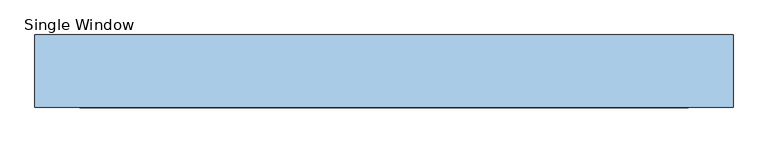
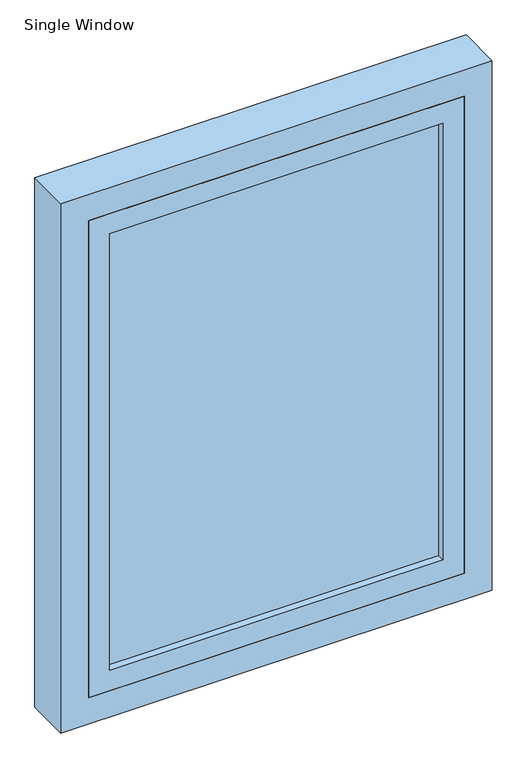
"""IFC4 building model written with IfcOpenShell, lengths in millimetres: window geometry, Single Window : 10x13 Inåtgående."""

from ifc_helpers import new_model, si_unit, frame, origin, place, context, project, spatial, polyline, outline, extrude, source, transform, mapped, element, save


def single_window_e1c0cfdf(model_context):
    return source(origin(), model_context, "Body", "SweptSolid", [
        extrude(outline(polyline([(510.0, -6.75), (-370.0, -6.75), (-370.0, 9.25), (510.0, 9.25), (510.0, -6.75)])), frame((0.0, 0.0, 865.0), z_axis=(0.0, 0.0, 1.0), x_axis=(1.0, 0.0, 0.0)), (0.0, 0.0, 1.0), 1180.0),
        extrude(outline(polyline([(2045.0, 510.0), (2045.0, -370.0), (865.0, -370.0), (865.0, 510.0), (2045.0, 510.0)]), holes=[polyline([(915.0, 460.0), (915.0, -320.0), (1995.0, -320.0), (1995.0, 460.0), (915.0, 460.0)])]), frame((0.0, -25.0, 0.0), z_axis=(0.0, 1.0, 0.0), x_axis=(0.0, 0.0, 1.0)), (0.0, 0.0, 1.0), 52.5),
        extrude(outline(polyline([(800.0, -435.0), (800.0, 575.0), (2110.0, 575.0), (2110.0, -435.0), (800.0, -435.0)]), holes=[polyline([(865.0, 510.0), (865.0, -370.0), (2045.0, -370.0), (2045.0, 510.0), (865.0, 510.0)])]), frame((0.0, -25.0, 0.0), z_axis=(0.0, 1.0, 0.0), x_axis=(0.0, 0.0, 1.0)), (0.0, 0.0, 1.0), 105.0),
    ])


if __name__ == "__main__":
    model = new_model("IFC4")
    model_context = context("Model", 3, world=origin())
    ifc_project = project(units=[si_unit("LENGTHUNIT", "METRE", prefix="MILLI")], contexts=[model_context])
    site = spatial("IfcSite", under=ifc_project)
    building = spatial("IfcBuilding", under=site)
    placement = place(None, origin())
    single_window_shape = single_window_e1c0cfdf(model_context)
    element("IfcWindow", 1, ObjectType="Single Window : 10x13 Inåtgående", at=placement, inside=building, context=model_context, shape_type="MappedRepresentation", body=[
        mapped(single_window_shape, transform((0.0, 0.0, 0.0), x_axis=(1.0, 0.0, 0.0), y_axis=(0.0, 1.0, 0.0), z_axis=(0.0, 0.0, 1.0))),
    ])
    save(model, "model.ifc")

# Revit data of these elements
# Type "Single Window : 10x13 Inåtgående"
#   Type Mark = "F2"
#   CQSwingCount = ""
#   URL = "www.cad-q.se"
#   Keynote = "42.D"
#   Construction Type = "Generellt fönster"
#   CQOriginalSwingDirection = "Left"
#   Analytic Construction = "<None>"
#   Wall Width [instance default] = 350 mm
#   Rough Width = 1010 mm
#   Rough Height = 1310 mm
#   Inset1000 [instance default] = 1070 mm
#   Inset [instance default] = 70 mm
#   Height [instance default] = 1310 mm
#   GapTop [instance default] = 15 mm
#   GapSecondary [instance default] = 15 mm
#   GapPrimary [instance default] = 15 mm
#   GapBottom [instance default] = 15 mm
#   Gap = 15 mm
#   Frame Width = 980 mm
#   Frame Thickness = 50 mm
#   Frame Height = 1280 mm
#   Frame Depth = 105 mm
#   Width [instance default] = 1010 mm
#   Default Sill Height = 800 mm
#   Panel Height = 1180 mm
#   Panel Width = 880 mm
#   MWidth [instance default] = 10
#   MHeight [instance default] = 13
#   Gap Top [instance default] = yes
#   Gap Secondary Side [instance default] = yes
#   Gap Primary Side [instance default] = yes
#   Gap Bottom [instance default] = yes
#   Material Interior = Default Window Interior
#   Material Glass = none
#   Material Exterior = none
#   Panel Operation = element 308022
#   Wall Closure = (empty or 0)
#   Assembly Code = ""
# Element 1 (IfcWindow, "Single Window : 10x13 Inåtgående")
#   Wall Width = 300 mm
#   Materials on its faces: "Partier - Generell", "Glas - Generellt", "Default Window Interior"
# Materials
#   "Default Window Interior": class "Paint", colour RGB 255 255 255, transparency 0, URL = "www.cad-q.se", Description = "Målning", Cost = 0
#   "Partier - Generell": class "Generic", colour RGB 153 153 153, transparency 0, URL = "www.cad-q.se", Description = "Odefinierat material", Cost = 0
#   "Glas - Generellt": class "Generic", colour RGB 159 197 217, transparency 0.9, URL = "www.cad-q.se", Description = "Odefinerat Glas", Cost = 0
